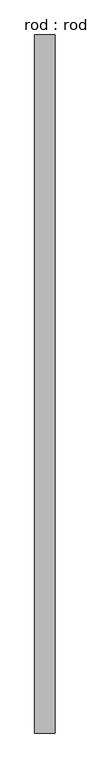
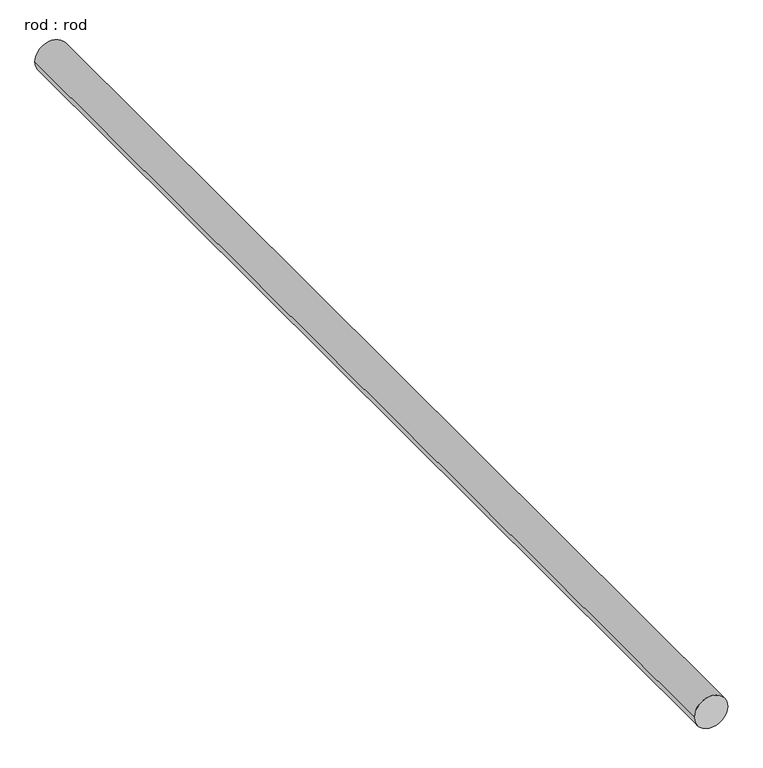
"""IFC4 building model written with IfcOpenShell, lengths in millimetres: proxy geometry, rod : rod."""

from ifc_helpers import new_model, si_unit, point, frame, frame_2d, origin, place, context, project, spatial, circle_curve, trimmed, segment, composite_curve, outline, extrude, source, transform, mapped, element, save


def rod_rod_d9c04cca(model_context):
    return source(origin(), model_context, "Body", "SweptSolid", [
        extrude(outline(composite_curve([segment(trimmed(circle_curve(frame_2d((0.0108462, 0.0)), 200.0), [point((0.0108462, 200.0))], [point((0.0108462, -200.0))], False, "CARTESIAN"), True, "CONTINUOUS"), segment(trimmed(circle_curve(frame_2d((0.0108462, 0.0)), 200.0), [point((0.0108462, -200.0))], [point((0.0108462, 200.0))], False, "CARTESIAN"), True, "CONTINUOUS")], self_intersect=False)), frame((0.0, -2740.604718, 0.0), z_axis=(0.0, 1.0, 0.0), x_axis=(0.0, 0.0, 1.0)), (0.0, 0.0, 1.0), 13666.6666667),
    ])


if __name__ == "__main__":
    model = new_model("IFC4")
    model_context = context("Model", 3, world=origin())
    ifc_project = project(units=[si_unit("LENGTHUNIT", "METRE", prefix="MILLI")], contexts=[model_context])
    site = spatial("IfcSite", under=ifc_project)
    building = spatial("IfcBuilding", under=site)
    placement = place(None, origin())
    rod_rod_shape = rod_rod_d9c04cca(model_context)
    element("IfcBuildingElementProxy", 1, Name="rod : rod", ObjectType="rod : rod", at=placement, inside=building, context=model_context, shape_type="MappedRepresentation", body=[
        mapped(rod_rod_shape, transform((0.0, 0.0, 0.0), x_axis=(1.0, 0.0, 0.0), y_axis=(0.0, 1.0, 0.0), z_axis=(0.0, 0.0, 1.0))),
    ])
    save(model, "model.ifc")

# Revit data of these elements
# Type "rod : rod"
#   Default Elevation = 0
